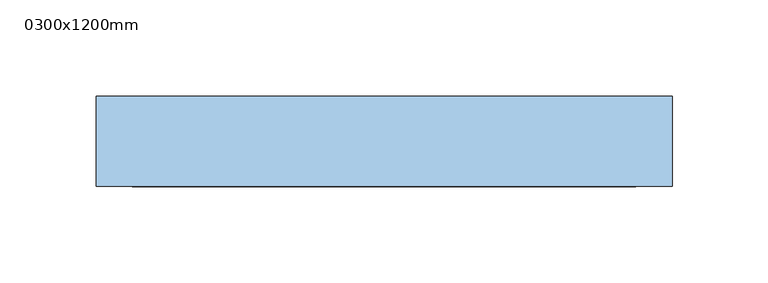
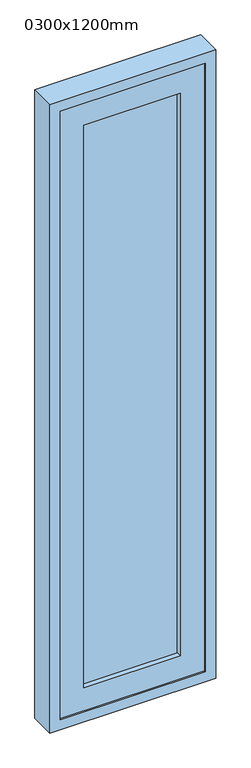
"""IFC4 building model written with IfcOpenShell, lengths in millimetres: window geometry, Janela Pivotante : 0300x1200mm."""

from ifc_helpers import new_model, si_unit, frame, origin, place, context, project, spatial, polyline, outline, extrude, source, transform, mapped, element, save


def window_0300x1200mm_6bc9c297(model_context):
    return source(origin(), model_context, "Body", "SweptSolid", [
        extrude(outline(polyline([(-87.0, -86.1), (-87.0, -81.1), (87.0, -81.1), (87.0, -86.1), (-87.0, -86.1)])), frame((0.0, 0.0, 563.0), z_axis=(0.0, 0.0, 1.0), x_axis=(1.0, 0.0, 0.0)), (0.0, 0.0, 1.0), 1074.0),
        extrude(outline(polyline([(1681.0, -131.0), (519.0, -131.0), (519.0, 131.0), (1681.0, 131.0), (1681.0, -131.0)]), holes=[polyline([(1637.0, -87.0), (1637.0, 87.0), (563.0, 87.0), (563.0, -87.0), (1637.0, -87.0)])]), frame((0.0, -95.6, 0.0), z_axis=(0.0, 1.0, 0.0), x_axis=(0.0, 0.0, 1.0)), (0.0, 0.0, 1.0), 24.0),
        extrude(outline(polyline([(1700.0, -150.0), (500.0, -150.0), (500.0, 150.0), (1700.0, 150.0), (1700.0, -150.0)]), holes=[polyline([(1681.0, -131.0), (1681.0, 131.0), (519.0, 131.0), (519.0, -131.0), (1681.0, -131.0)])]), frame((0.0, -98.6, 0.0), z_axis=(0.0, 1.0, 0.0), x_axis=(0.0, 0.0, 1.0)), (0.0, 0.0, 1.0), 47.0),
    ])


if __name__ == "__main__":
    model = new_model("IFC4")
    model_context = context("Model", 3, world=origin())
    ifc_project = project(units=[si_unit("LENGTHUNIT", "METRE", prefix="MILLI")], contexts=[model_context])
    site = spatial("IfcSite", under=ifc_project)
    building = spatial("IfcBuilding", under=site)
    placement = place(None, origin())
    window_0300x1200mm_shape = window_0300x1200mm_6bc9c297(model_context)
    element("IfcWindow", 1, ObjectType="Janela Pivotante : 0300x1200mm", at=placement, inside=building, context=model_context, shape_type="MappedRepresentation", body=[
        mapped(window_0300x1200mm_shape, transform((0.0, 0.0, 0.0), x_axis=(1.0, 0.0, 0.0), y_axis=(0.0, 1.0, 0.0), z_axis=(0.0, 0.0, 1.0))),
    ])
    save(model, "model.ifc")

# Revit data of these elements
# Type "Janela Pivotante : 0300x1200mm"
#   Type Mark = ""
#   SINAPI = ""
#   Módulo Básico M = 10.00 cm
#   Largura de Coordenação Modular CM = 30.00 cm
#   Rough Width = 30.00 cm
#   Espessura Painel = 2.40 cm
#   Altura de Coordenação Modular = 120.00 cm
#   Rough Height = 120.00 cm
#   Height = 120.00 cm
#   Altura Peitoril = 50.00 cm
#   Width = 30.00 cm
#   Ajuste de Coordenação Modular AC = 0.00 cm
#   Número de Módulos Básicos nM Largura = 3
#   Número de Módulos Básicos nM Altura = 12
#   Marco = Metal - Alumínio
#   Painel = Vidro
#   Assembly Code = ""
#   Wall Closure = (empty or 0)
# Element 1 (IfcWindow, "Janela Pivotante : 0300x1200mm")
#   Materials on its faces: "Metal - Alumínio", "Vidro"
# Materials
#   "Metal - Alumínio": class "Metal", colour RGB 244 244 244, transparency 0
#   "Vidro": class "Vidro", colour RGB 230 230 230, transparency 0.75, Cost = 0
